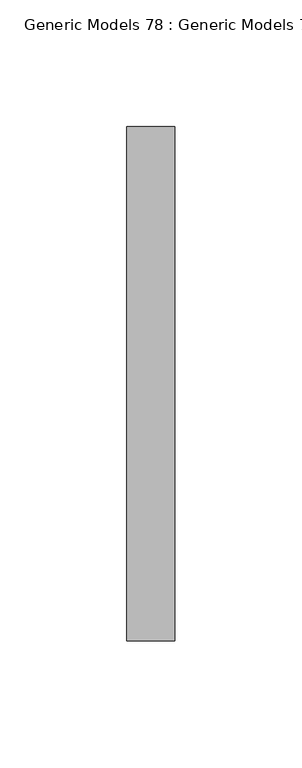
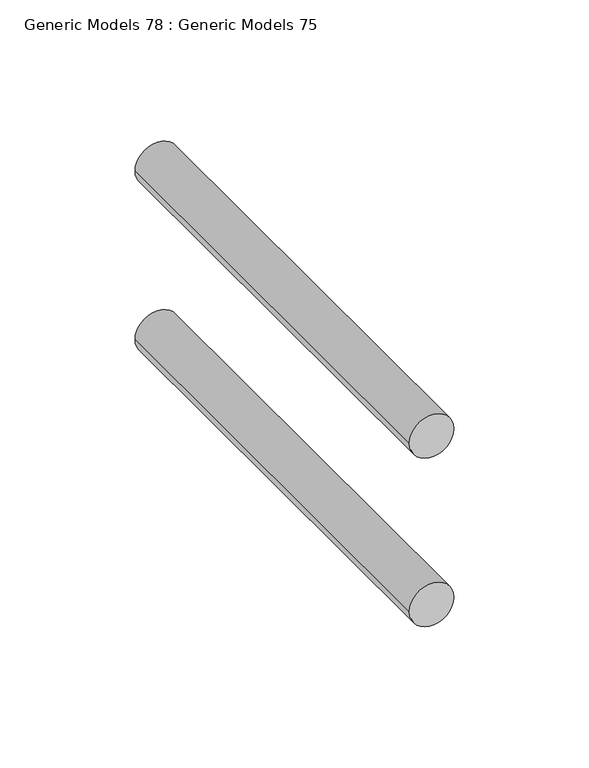
"""IFC4 building model written with IfcOpenShell, lengths in millimetres: proxy geometry, Generic Models 78 : Generic Models 75."""

from ifc_helpers import new_model, si_unit, point, frame, frame_2d, origin, place, context, project, spatial, circle_curve, trimmed, segment, composite_curve, outline, extrude, source, transform, mapped, element, save


def generic_models_78_generic_models_75_761e1f1d(model_context):
    return source(origin(), model_context, "Body", "SweptSolid", [
        extrude(outline(composite_curve([segment(trimmed(circle_curve(frame_2d((271267.2375, 31975.4096032)), 9.525), [point((271267.2375, 31965.8846032))], [point((271267.2375, 31984.9346032))], False, "CARTESIAN"), True, "CONTINUOUS"), segment(trimmed(circle_curve(frame_2d((271267.2375, 31975.4096032)), 9.525), [point((271267.2375, 31984.9346032))], [point((271267.2375, 31965.8846032))], False, "CARTESIAN"), True, "CONTINUOUS")], self_intersect=False)), frame((0.0, 30672.7406612, 0.0), z_axis=(0.0, 1.0, 0.0), x_axis=(0.0, 0.0, 1.0)), (0.0, 0.0, 1.0), 203.2),
        extrude(outline(composite_curve([segment(trimmed(circle_curve(frame_2d((271343.4375, 31975.4096032)), 9.525), [point((271343.4375, 31965.8846032))], [point((271343.4375, 31984.9346032))], False, "CARTESIAN"), True, "CONTINUOUS"), segment(trimmed(circle_curve(frame_2d((271343.4375, 31975.4096032)), 9.525), [point((271343.4375, 31984.9346032))], [point((271343.4375, 31965.8846032))], False, "CARTESIAN"), True, "CONTINUOUS")], self_intersect=False)), frame((0.0, 30672.7406612, 0.0), z_axis=(0.0, 1.0, 0.0), x_axis=(0.0, 0.0, 1.0)), (0.0, 0.0, 1.0), 203.2),
    ])


if __name__ == "__main__":
    model = new_model("IFC4")
    model_context = context("Model", 3, world=origin())
    ifc_project = project(units=[si_unit("LENGTHUNIT", "METRE", prefix="MILLI")], contexts=[model_context])
    site = spatial("IfcSite", under=ifc_project)
    building = spatial("IfcBuilding", under=site)
    placement = place(None, origin())
    generic_models_78_generic_models_75_shape = generic_models_78_generic_models_75_761e1f1d(model_context)
    element("IfcBuildingElementProxy", 1, Name="Generic Models 78 : Generic Models 75", ObjectType="Generic Models 78 : Generic Models 75", at=placement, inside=building, context=model_context, shape_type="MappedRepresentation", body=[
        mapped(generic_models_78_generic_models_75_shape, transform((0.0, 0.0, 0.0), x_axis=(1.0, 0.0, 0.0), y_axis=(0.0, 1.0, 0.0), z_axis=(0.0, 0.0, 1.0))),
    ])
    save(model, "model.ifc")
